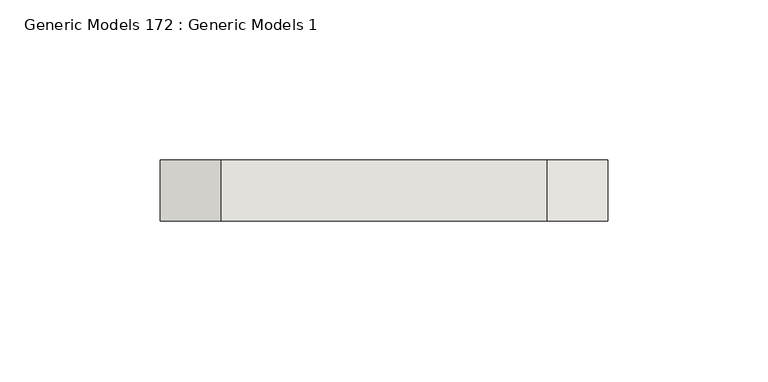
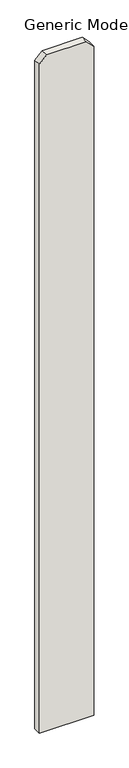
"""IFC4 building model written with IfcOpenShell, lengths in millimetres: wall geometry, Generic Models 172 : Generic Models 1."""

from ifc_helpers import new_model, si_unit, frame, origin, place, context, project, spatial, polyline, outline, extrude, source, transform, mapped, element, save


def generic_models_172_generic_models_1_03810ec6(model_context):
    return source(origin(), model_context, "Body", "SweptSolid", [
        extrude(outline(polyline([(76.2, 325194.6125), (1885.95, 325194.6125), (1905.0, 325175.5625), (1905.0, 325073.9625), (1885.95, 325054.9125), (76.2, 325054.9125), (76.2, 325194.6125)])), frame((0.0, 547.6875, 0.0), z_axis=(0.0, 1.0, 0.0), x_axis=(0.0, 0.0, 1.0)), (0.0, 0.0, 1.0), 19.05),
    ])


if __name__ == "__main__":
    model = new_model("IFC4")
    model_context = context("Model", 3, world=origin())
    ifc_project = project(units=[si_unit("LENGTHUNIT", "METRE", prefix="MILLI")], contexts=[model_context])
    site = spatial("IfcSite", under=ifc_project)
    building = spatial("IfcBuilding", under=site)
    placement = place(None, origin())
    generic_models_172_generic_models_1_shape = generic_models_172_generic_models_1_03810ec6(model_context)
    element("IfcWall", 1, ObjectType="Generic Models 172 : Generic Models 1", at=placement, inside=building, context=model_context, shape_type="MappedRepresentation", body=[
        mapped(generic_models_172_generic_models_1_shape, transform((0.0, 0.0, 0.0), x_axis=(1.0, 0.0, 0.0), y_axis=(0.0, 1.0, 0.0), z_axis=(0.0, 0.0, 1.0))),
    ])
    save(model, "model.ifc")

# Revit data of these elements
# Element 1 (IfcWall, "Generic Models 172 : Generic Models 1")
#   Materials on its faces: "VERTICAL 1X6 CEDAR PLANKS W/ CLEAR WOOD SEALER"
# Materials
#   "VERTICAL 1X6 CEDAR PLANKS W/ CLEAR WOOD SEALER": class "Wood", colour RGB 234 198 147, transparency 0, Description = "Pinus Echinata", Cost = 0
